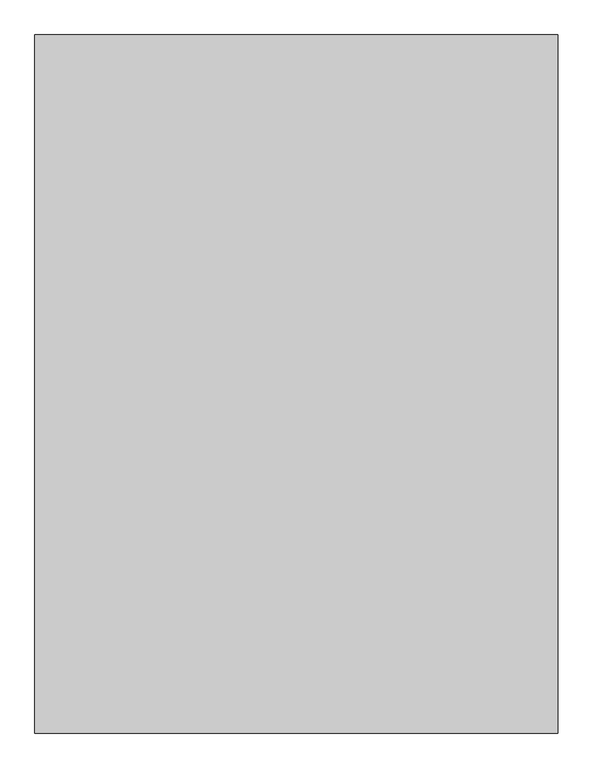
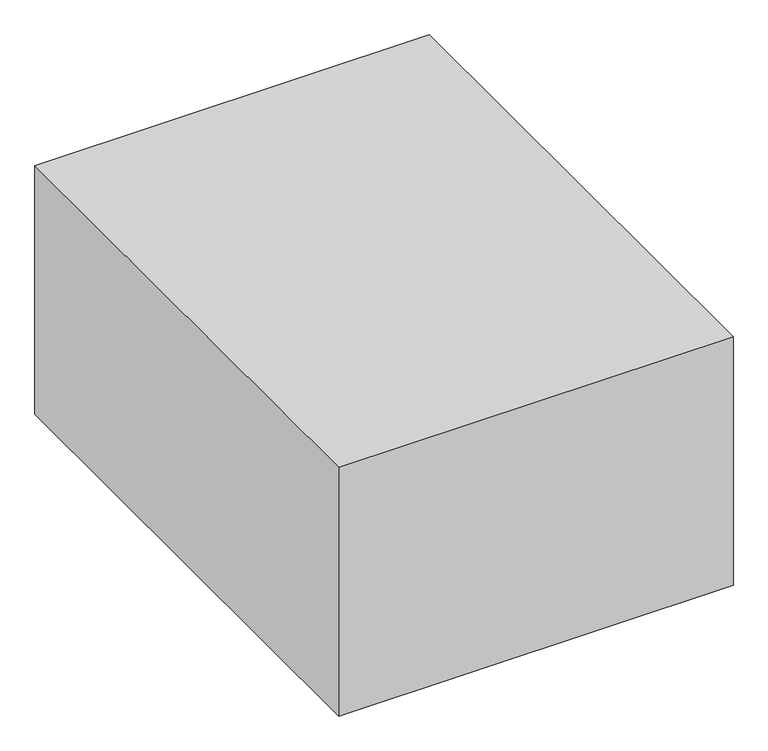
"""IFC4 building model written with IfcOpenShell, lengths in millimetres: proxy geometry, Space Planning Box_hec : Space Planning Box_hec."""

from ifc_helpers import new_model, si_unit, origin, origin_with_axes, place, context, project, spatial, polyline, outline, extrude, source, transform, mapped, element, save


def generic_models_399a6151(model_context):
    return source(origin(), model_context, "Body", "SweptSolid", [
        extrude(outline(polyline([(4500.0, 6000.0), (4500.0, -6000.0), (-4500.0, -6000.0), (-4500.0, 6000.0), (4500.0, 6000.0)])), origin_with_axes(), (0.0, 0.0, 1.0), 6000.0),
    ])


if __name__ == "__main__":
    model = new_model("IFC4")
    model_context = context("Model", 3, world=origin())
    ifc_project = project(units=[si_unit("LENGTHUNIT", "METRE", prefix="MILLI")], contexts=[model_context])
    site = spatial("IfcSite", under=ifc_project)
    building = spatial("IfcBuilding", under=site)
    placement = place(None, origin())
    generic_models_shape = generic_models_399a6151(model_context)
    element("IfcBuildingElementProxy", 1, Name="Space Planning Box_hec : Space Planning Box_hec", ObjectType="Space Planning Box_hec : Space Planning Box_hec", at=placement, inside=building, context=model_context, shape_type="MappedRepresentation", body=[
        mapped(generic_models_shape, transform((0.0, 0.0, 0.0), x_axis=(1.0, 0.0, 0.0), y_axis=(0.0, 1.0, 0.0), z_axis=(0.0, 0.0, 1.0))),
    ])
    save(model, "model.ifc")

# Revit data of these elements
# Type "Space Planning Box_hec : Space Planning Box_hec"
#   Type Comments = "..."
#   Room Name [instance default] = "?"
#   Interior Finish [instance default] = ""
#   Exterior Finish [instance default] = ""
#   Department [instance default] = ""
#   Assembly Code = "..."
#   Width [instance default] = 1524 mm
#   Program Area [instance default] = 0.00 m²
#   Length [instance default] = 1524 mm
#   Height [instance default] = 1524 mm
#   Area [instance default] = 2.32258 m²
#   Fill Color [instance default] = Cyan
#   Default Elevation = 0
# Element 1 (IfcBuildingElementProxy, "Space Planning Box_hec : Space Planning Box_hec")
#   Room Name = "Battery Room"
#   Interior Finish = "IF4"
#   Exterior Finish = "EF1"
#   Department = "EL"
#   Width = 9000 mm
#   Program Area = 108.00 m²
#   Length = 12000 mm
#   Height = 6000 mm
#   Area = 108.00 m²
#   Fill Color = Blue
#   Materials on its faces: "Blue"
# Materials
#   "Cyan": class "Generic", colour RGB 0 255 255, transparency 0.2, Cost = 0
#   "Blue": class "Generic", colour RGB 0 0 255, transparency 0.2, Cost = 0
